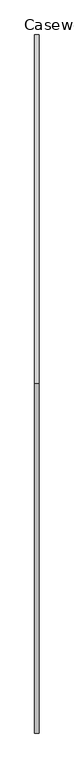
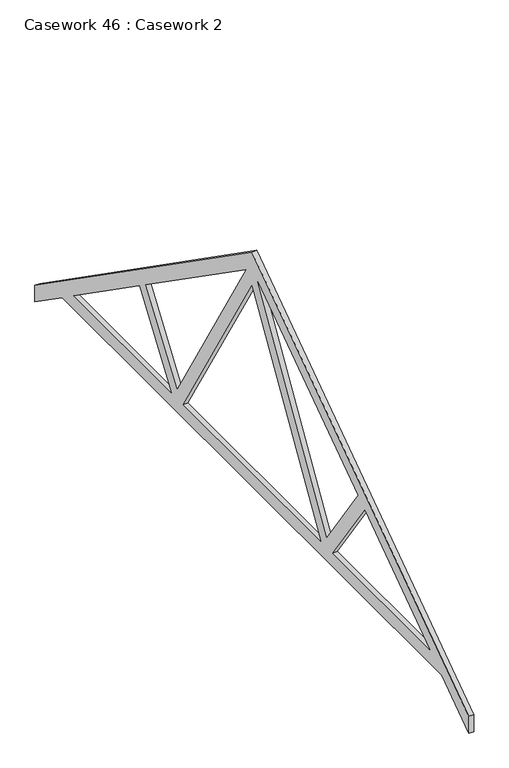
"""IFC4 building model written with IfcOpenShell, lengths in millimetres: furniture geometry, Casework 46 : Casework 2."""

import ifcopenshell
import ifcopenshell.guid

model = None  # the IFC model being written
_history = None  # IfcOwnerHistory: only IFC2X3 demands one
_inside = {}  # id of a spatial element -> (the spatial element, [elements in it])
_under = {}  # id of a project, library or spatial element -> (it, [spatial elements below it])
_declared = {}  # id of a project -> (the project, [libraries it declares])
_typed = {}  # id of a type object -> (the type object, [elements of that type])
_made_of = {}  # id of a material, layer set ... -> (it, [elements and type objects made of it])


def new_model(schema):
    """Start an empty IFC model of exactly this schema.

    Asked for "IFC4X3", IfcOpenShell would pick the latest addendum, in which some entities
    have other attributes; the version numbers below select the first issue.
    IFC2X3 requires an IfcOwnerHistory on every rooted entity: one is made here for all.
    """
    global model, _history
    if schema == "IFC4X3":
        model = ifcopenshell.file(schema_version=(4, 3, 0, 0))
    else:
        model = ifcopenshell.file(schema=schema)
    _inside.clear()
    _under.clear()
    _declared.clear()
    _typed.clear()
    _made_of.clear()
    _history = None
    if model.schema == "IFC2X3":
        org = make("IfcOrganization", Name="unknown")
        user = make(
            "IfcPersonAndOrganization",
            ThePerson=make("IfcPerson", FamilyName="unknown"),
            TheOrganization=org,
        )
        app = make(
            "IfcApplication",
            ApplicationDeveloper=org,
            Version="unknown",
            ApplicationFullName="unknown",
            ApplicationIdentifier="unknown",
        )
        _history = make(
            "IfcOwnerHistory",
            OwningUser=user,
            OwningApplication=app,
            ChangeAction="ADDED",
            CreationDate=0,
        )
    return model


def make(cls, **values):
    """One entity of the class cls with the attributes given. An attribute that is None is left unset."""
    return model.create_entity(
        cls, **{name: value for name, value in values.items() if value is not None}
    )


def rooted(cls, **values):
    """An entity with a GlobalId (a new one), such as an element, a storey or a relation."""
    return make(cls, GlobalId=ifcopenshell.guid.new(), OwnerHistory=_history, **values)


def si_unit(unit_type, name, prefix=None):
    """IfcSIUnit, for example si_unit("LENGTHUNIT", "METRE", prefix="MILLI")."""
    return make("IfcSIUnit", UnitType=unit_type, Prefix=prefix, Name=name)


def assignment(units):
    """IfcUnitAssignment: the units of a project."""
    return None if units is None else make("IfcUnitAssignment", Units=units)


def point(xyz):
    """IfcCartesianPoint."""
    return None if xyz is None else make("IfcCartesianPoint", Coordinates=xyz)


def direction(xyz):
    """IfcDirection."""
    return None if xyz is None else make("IfcDirection", DirectionRatios=xyz)


def frame(location, z_axis=None, x_axis=None):
    """IfcAxis2Placement3D, a coordinate frame: its origin and axes. An axis left out is left unset."""
    return make(
        "IfcAxis2Placement3D",
        Location=point(location),
        Axis=direction(z_axis),
        RefDirection=direction(x_axis),
    )


def origin():
    """The frame at (0, 0, 0) with its axes left unset."""
    return frame((0.0, 0.0, 0.0))


def place(relative_to, where):
    """IfcLocalPlacement: puts the frame where relative to a parent placement (None: the world)."""
    return make(
        "IfcLocalPlacement", PlacementRelTo=relative_to, RelativePlacement=where
    )


def context(
    kind, dimensions, precision=None, world=None, true_north=None, identifier=None
):
    """IfcGeometricRepresentationContext, for example the 3D "Model" context."""
    return make(
        "IfcGeometricRepresentationContext",
        ContextIdentifier=identifier,
        ContextType=kind,
        CoordinateSpaceDimension=dimensions,
        Precision=precision,
        WorldCoordinateSystem=world,
        TrueNorth=true_north,
    )


def project(units=None, contexts=None):
    """IfcProject with its units and contexts."""
    return rooted(
        "IfcProject",
        Name="project",
        RepresentationContexts=contexts,
        UnitsInContext=assignment(units),
    )


def spatial(cls, under=None, at=None, **own):
    """A site, building, storey or space (cls), placed at a placement, below another one or the project."""
    s = rooted(cls, ObjectPlacement=at, **own)
    if under is not None:
        _under.setdefault(under.id(), (under, []))[1].append(s)
    return s


def polyline(points):
    """IfcPolyline through the points."""
    return make("IfcPolyline", Points=[point(p) for p in points])


def outline(outer, holes=None, kind="AREA"):
    """IfcArbitraryClosedProfileDef: a profile drawn as a closed curve; with holes, ...WithVoids."""
    if holes is None:
        return make("IfcArbitraryClosedProfileDef", ProfileType=kind, OuterCurve=outer)
    return make(
        "IfcArbitraryProfileDefWithVoids",
        ProfileType=kind,
        OuterCurve=outer,
        InnerCurves=holes,
    )


def extrude(swept, where, along, depth):
    """IfcExtrudedAreaSolid: the profile swept, set in the frame where, extruded along a direction by depth."""
    return make(
        "IfcExtrudedAreaSolid",
        SweptArea=swept,
        Position=where,
        ExtrudedDirection=direction(along),
        Depth=depth,
    )


def shape(context_of_items, identifier, shape_type, items):
    """IfcShapeRepresentation: the items that make up one representation, for example the "Body"."""
    return make(
        "IfcShapeRepresentation",
        ContextOfItems=context_of_items,
        RepresentationIdentifier=identifier,
        RepresentationType=shape_type,
        Items=items,
    )


def source(mapping_origin, context_of_items, identifier, shape_type, items):
    """IfcRepresentationMap: a shape defined once, which mapped items show again and again."""
    return make(
        "IfcRepresentationMap",
        MappingOrigin=mapping_origin,
        MappedRepresentation=shape(context_of_items, identifier, shape_type, items),
    )


def transform(
    local_origin,
    x_axis=None,
    y_axis=None,
    z_axis=None,
    scale=None,
    scale2=None,
    scale3=None,
    uniform=True,
):
    """IfcCartesianTransformationOperator3D, or its non-uniform kind. x_axis, y_axis, z_axis: its Axis1, 2, 3."""
    if uniform:
        return make(
            "IfcCartesianTransformationOperator3D",
            Axis1=direction(x_axis),
            Axis2=direction(y_axis),
            LocalOrigin=point(local_origin),
            Scale=scale,
            Axis3=direction(z_axis),
        )
    return make(
        "IfcCartesianTransformationOperator3DnonUniform",
        Axis1=direction(x_axis),
        Axis2=direction(y_axis),
        LocalOrigin=point(local_origin),
        Scale=scale,
        Axis3=direction(z_axis),
        Scale2=scale2,
        Scale3=scale3,
    )


def mapped(mapping_source, mapping_target):
    """IfcMappedItem: shows the shape of a source again, moved by a transform."""
    return make(
        "IfcMappedItem", MappingSource=mapping_source, MappingTarget=mapping_target
    )


def made_of(thing, what):
    """Note that an element or type object is made of a material, layer set ...; save() writes the relation."""
    if what is not None:
        _made_of.setdefault(what.id(), (what, []))[1].append(thing)
    return thing


def element(
    cls,
    number,
    at=None,
    inside=None,
    cuts=None,
    type_object=None,
    material=None,
    context=None,
    identifier="Body",
    shape_type=None,
    held_by="IfcProductDefinitionShape",
    body=None,
    shapes=None,
    **own,
):
    """One element of the class cls, such as IfcWall. Its Tag is "e" and its number.

    at: its placement. inside: the storey or other place that contains it. cuts: it is an
    opening in that element (IfcRelVoidsElement). A single representation is given by context,
    identifier, shape_type and body (its items); several are given by shapes. held_by: the class
    of the entity that holds the representations. save() writes the other relations.
    """
    e = rooted(cls, Tag="e%d" % number, ObjectPlacement=at, **own)
    if body is not None:
        shapes = [shape(context, identifier, shape_type, body)]
    if shapes is not None:
        e.Representation = make(held_by, Representations=shapes)
    if inside is not None:
        _inside.setdefault(inside.id(), (inside, []))[1].append(e)
    if cuts is not None:
        rooted(
            "IfcRelVoidsElement", RelatingBuildingElement=cuts, RelatedOpeningElement=e
        )
    if type_object is not None:
        _typed.setdefault(type_object.id(), (type_object, []))[1].append(e)
    return made_of(e, material)


def aggregate(whole, parts):
    """IfcRelAggregates: a whole, such as a stair, and the parts it consists of."""
    return rooted("IfcRelAggregates", RelatingObject=whole, RelatedObjects=parts)


def save(model, path):
    """Write the relations noted so far, then the file.

    IfcRelAggregates (storeys below a building ...), IfcRelContainedInSpatialStructure (elements
    in a storey), IfcRelDefinesByType, IfcRelAssociatesMaterial and IfcRelDeclares: one each for
    every whole, place, type object, material and project.
    """
    for whole, parts in _under.values():
        aggregate(whole, parts)
    for where, things in _inside.values():
        rooted(
            "IfcRelContainedInSpatialStructure",
            RelatedElements=things,
            RelatingStructure=where,
        )
    for kind, things in _typed.values():
        rooted("IfcRelDefinesByType", RelatedObjects=things, RelatingType=kind)
    for what, things in _made_of.values():
        rooted("IfcRelAssociatesMaterial", RelatedObjects=things, RelatingMaterial=what)
    for by, libraries in _declared.values():
        rooted("IfcRelDeclares", RelatingContext=by, RelatedDefinitions=libraries)
    model.write(path)


def casework_46_casework_2_9ef60b2c(model_context):
    return source(origin(), model_context, "Body", "SweptSolid", [
        extrude(outline(polyline([(6583.1149316, 5250.0), (-277.3850684, 5250.0), (-767.3850684, 4906.8983063), (-767.3850684, 5090.0144946), (3152.8649316, 7835.0030963), (7073.1149316, 5090.0144946), (7073.1149316, 4906.8983063), (6583.1149316, 5250.0)]), holes=[polyline([(4612.3149663, 5400.0), (6368.8927306, 5400.0), (5190.2113591, 6225.3215815), (4612.3149663, 5400.0)]), polyline([(4394.2037684, 5400.0), (3152.8649316, 7465.9347567), (1911.5260948, 5400.0), (4394.2037684, 5400.0)]), polyline([(4504.5438357, 5507.6038939), (5067.3385525, 6311.3580469), (3262.0771677, 7575.415677), (4504.5438357, 5507.6038939)]), polyline([(1693.4148969, 5400.0), (1115.5185041, 6225.3215815), (-63.1628674, 5400.0), (1693.4148969, 5400.0)]), polyline([(1801.1860276, 5507.6038939), (3043.6526956, 7575.415677), (1238.3913108, 6311.3580469), (1801.1860276, 5507.6038939)])]), frame((-10421.5247381, 0.0, 0.0), z_axis=(1.0, 0.0, 0.0), x_axis=(0.0, 1.0, 0.0)), (0.0, 0.0, 1.0), 49.6351915),
    ])


if __name__ == "__main__":
    model = new_model("IFC4")
    model_context = context("Model", 3, world=origin())
    ifc_project = project(units=[si_unit("LENGTHUNIT", "METRE", prefix="MILLI")], contexts=[model_context])
    site = spatial("IfcSite", under=ifc_project)
    building = spatial("IfcBuilding", under=site)
    placement = place(None, origin())
    casework_46_casework_2_shape = casework_46_casework_2_9ef60b2c(model_context)
    element("IfcFurniture", 1, ObjectType="Casework 46 : Casework 2", at=placement, inside=building, context=model_context, shape_type="MappedRepresentation", body=[
        mapped(casework_46_casework_2_shape, transform((0.0, 0.0, 0.0), x_axis=(1.0, 0.0, 0.0), y_axis=(0.0, 1.0, 0.0), z_axis=(0.0, 0.0, 1.0))),
    ])
    save(model, "model.ifc")

# Revit data of these elements
# Type "Casework 46 : Casework 2"
#   Manufacturer = "M W Roofs"
#   Type Comments = "Gangnail Roof Truss"
#   Finish = "Rough"
#   Construction Type = "Timber"
# Element 1 (IfcFurniture, "Casework 46 : Casework 2")
#   Materials on its faces: "Softwood, Lumber"
# Materials
#   "Softwood, Lumber": class "Wood", colour RGB 205 156 65, transparency 0, Description = "Pinus Echinata", Cost = 0
